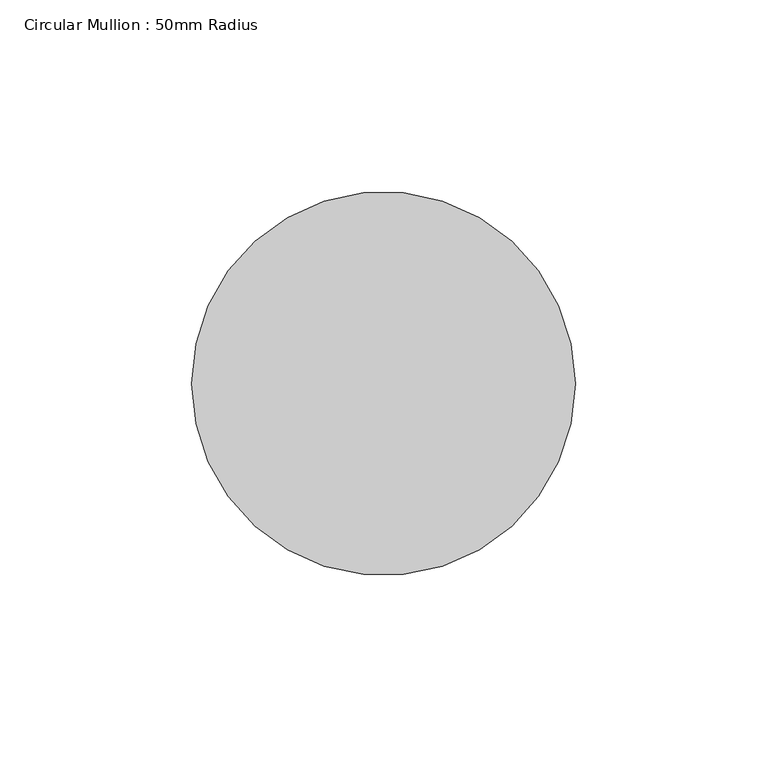
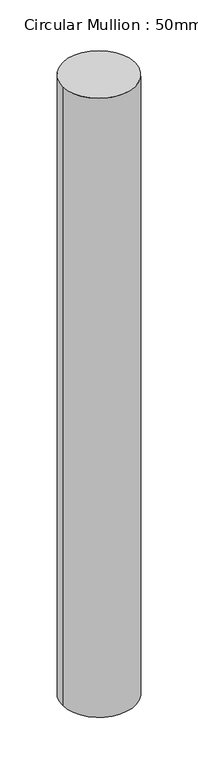
"""IFC4 building model written with IfcOpenShell, lengths in millimetres: member geometry, Circular Mullion : 50mm Radius."""

import ifcopenshell
import ifcopenshell.guid

model = None  # the IFC model being written
_history = None  # IfcOwnerHistory: only IFC2X3 demands one
_inside = {}  # id of a spatial element -> (the spatial element, [elements in it])
_under = {}  # id of a project, library or spatial element -> (it, [spatial elements below it])
_declared = {}  # id of a project -> (the project, [libraries it declares])
_typed = {}  # id of a type object -> (the type object, [elements of that type])
_made_of = {}  # id of a material, layer set ... -> (it, [elements and type objects made of it])


def new_model(schema):
    """Start an empty IFC model of exactly this schema.

    Asked for "IFC4X3", IfcOpenShell would pick the latest addendum, in which some entities
    have other attributes; the version numbers below select the first issue.
    IFC2X3 requires an IfcOwnerHistory on every rooted entity: one is made here for all.
    """
    global model, _history
    if schema == "IFC4X3":
        model = ifcopenshell.file(schema_version=(4, 3, 0, 0))
    else:
        model = ifcopenshell.file(schema=schema)
    _inside.clear()
    _under.clear()
    _declared.clear()
    _typed.clear()
    _made_of.clear()
    _history = None
    if model.schema == "IFC2X3":
        org = make("IfcOrganization", Name="unknown")
        user = make(
            "IfcPersonAndOrganization",
            ThePerson=make("IfcPerson", FamilyName="unknown"),
            TheOrganization=org,
        )
        app = make(
            "IfcApplication",
            ApplicationDeveloper=org,
            Version="unknown",
            ApplicationFullName="unknown",
            ApplicationIdentifier="unknown",
        )
        _history = make(
            "IfcOwnerHistory",
            OwningUser=user,
            OwningApplication=app,
            ChangeAction="ADDED",
            CreationDate=0,
        )
    return model


def make(cls, **values):
    """One entity of the class cls with the attributes given. An attribute that is None is left unset."""
    return model.create_entity(
        cls, **{name: value for name, value in values.items() if value is not None}
    )


def rooted(cls, **values):
    """An entity with a GlobalId (a new one), such as an element, a storey or a relation."""
    return make(cls, GlobalId=ifcopenshell.guid.new(), OwnerHistory=_history, **values)


def si_unit(unit_type, name, prefix=None):
    """IfcSIUnit, for example si_unit("LENGTHUNIT", "METRE", prefix="MILLI")."""
    return make("IfcSIUnit", UnitType=unit_type, Prefix=prefix, Name=name)


def assignment(units):
    """IfcUnitAssignment: the units of a project."""
    return None if units is None else make("IfcUnitAssignment", Units=units)


def point(xyz):
    """IfcCartesianPoint."""
    return None if xyz is None else make("IfcCartesianPoint", Coordinates=xyz)


def direction(xyz):
    """IfcDirection."""
    return None if xyz is None else make("IfcDirection", DirectionRatios=xyz)


def frame(location, z_axis=None, x_axis=None):
    """IfcAxis2Placement3D, a coordinate frame: its origin and axes. An axis left out is left unset."""
    return make(
        "IfcAxis2Placement3D",
        Location=point(location),
        Axis=direction(z_axis),
        RefDirection=direction(x_axis),
    )


def frame_2d(location, x_axis=None):
    """IfcAxis2Placement2D, a coordinate frame in the plane: its origin and x axis."""
    return make(
        "IfcAxis2Placement2D", Location=point(location), RefDirection=direction(x_axis)
    )


def origin():
    """The frame at (0, 0, 0) with its axes left unset."""
    return frame((0.0, 0.0, 0.0))


def origin_2d():
    """The frame at (0, 0) in the plane with its x axis left unset."""
    return frame_2d((0.0, 0.0))


def place(relative_to, where):
    """IfcLocalPlacement: puts the frame where relative to a parent placement (None: the world)."""
    return make(
        "IfcLocalPlacement", PlacementRelTo=relative_to, RelativePlacement=where
    )


def context(
    kind, dimensions, precision=None, world=None, true_north=None, identifier=None
):
    """IfcGeometricRepresentationContext, for example the 3D "Model" context."""
    return make(
        "IfcGeometricRepresentationContext",
        ContextIdentifier=identifier,
        ContextType=kind,
        CoordinateSpaceDimension=dimensions,
        Precision=precision,
        WorldCoordinateSystem=world,
        TrueNorth=true_north,
    )


def project(units=None, contexts=None):
    """IfcProject with its units and contexts."""
    return rooted(
        "IfcProject",
        Name="project",
        RepresentationContexts=contexts,
        UnitsInContext=assignment(units),
    )


def spatial(cls, under=None, at=None, **own):
    """A site, building, storey or space (cls), placed at a placement, below another one or the project."""
    s = rooted(cls, ObjectPlacement=at, **own)
    if under is not None:
        _under.setdefault(under.id(), (under, []))[1].append(s)
    return s


def circle_curve(where, radius):
    """IfcCircle in the frame where."""
    return make("IfcCircle", Position=where, Radius=radius)


def trimmed(basis, trim1, trim2, sense, master):
    """IfcTrimmedCurve: the piece of a basis curve between two trims."""
    return make(
        "IfcTrimmedCurve",
        BasisCurve=basis,
        Trim1=trim1,
        Trim2=trim2,
        SenseAgreement=sense,
        MasterRepresentation=master,
    )


def segment(curve, same_sense, transition):
    """IfcCompositeCurveSegment."""
    return make(
        "IfcCompositeCurveSegment",
        Transition=transition,
        SameSense=same_sense,
        ParentCurve=curve,
    )


def composite_curve(segments, self_intersect=None):
    """IfcCompositeCurve: segments joined end to end."""
    return make("IfcCompositeCurve", Segments=segments, SelfIntersect=self_intersect)


def outline(outer, holes=None, kind="AREA"):
    """IfcArbitraryClosedProfileDef: a profile drawn as a closed curve; with holes, ...WithVoids."""
    if holes is None:
        return make("IfcArbitraryClosedProfileDef", ProfileType=kind, OuterCurve=outer)
    return make(
        "IfcArbitraryProfileDefWithVoids",
        ProfileType=kind,
        OuterCurve=outer,
        InnerCurves=holes,
    )


def extrude(swept, where, along, depth):
    """IfcExtrudedAreaSolid: the profile swept, set in the frame where, extruded along a direction by depth."""
    return make(
        "IfcExtrudedAreaSolid",
        SweptArea=swept,
        Position=where,
        ExtrudedDirection=direction(along),
        Depth=depth,
    )


def shape(context_of_items, identifier, shape_type, items):
    """IfcShapeRepresentation: the items that make up one representation, for example the "Body"."""
    return make(
        "IfcShapeRepresentation",
        ContextOfItems=context_of_items,
        RepresentationIdentifier=identifier,
        RepresentationType=shape_type,
        Items=items,
    )


def source(mapping_origin, context_of_items, identifier, shape_type, items):
    """IfcRepresentationMap: a shape defined once, which mapped items show again and again."""
    return make(
        "IfcRepresentationMap",
        MappingOrigin=mapping_origin,
        MappedRepresentation=shape(context_of_items, identifier, shape_type, items),
    )


def transform(
    local_origin,
    x_axis=None,
    y_axis=None,
    z_axis=None,
    scale=None,
    scale2=None,
    scale3=None,
    uniform=True,
):
    """IfcCartesianTransformationOperator3D, or its non-uniform kind. x_axis, y_axis, z_axis: its Axis1, 2, 3."""
    if uniform:
        return make(
            "IfcCartesianTransformationOperator3D",
            Axis1=direction(x_axis),
            Axis2=direction(y_axis),
            LocalOrigin=point(local_origin),
            Scale=scale,
            Axis3=direction(z_axis),
        )
    return make(
        "IfcCartesianTransformationOperator3DnonUniform",
        Axis1=direction(x_axis),
        Axis2=direction(y_axis),
        LocalOrigin=point(local_origin),
        Scale=scale,
        Axis3=direction(z_axis),
        Scale2=scale2,
        Scale3=scale3,
    )


def mapped(mapping_source, mapping_target):
    """IfcMappedItem: shows the shape of a source again, moved by a transform."""
    return make(
        "IfcMappedItem", MappingSource=mapping_source, MappingTarget=mapping_target
    )


def made_of(thing, what):
    """Note that an element or type object is made of a material, layer set ...; save() writes the relation."""
    if what is not None:
        _made_of.setdefault(what.id(), (what, []))[1].append(thing)
    return thing


def element(
    cls,
    number,
    at=None,
    inside=None,
    cuts=None,
    type_object=None,
    material=None,
    context=None,
    identifier="Body",
    shape_type=None,
    held_by="IfcProductDefinitionShape",
    body=None,
    shapes=None,
    **own,
):
    """One element of the class cls, such as IfcWall. Its Tag is "e" and its number.

    at: its placement. inside: the storey or other place that contains it. cuts: it is an
    opening in that element (IfcRelVoidsElement). A single representation is given by context,
    identifier, shape_type and body (its items); several are given by shapes. held_by: the class
    of the entity that holds the representations. save() writes the other relations.
    """
    e = rooted(cls, Tag="e%d" % number, ObjectPlacement=at, **own)
    if body is not None:
        shapes = [shape(context, identifier, shape_type, body)]
    if shapes is not None:
        e.Representation = make(held_by, Representations=shapes)
    if inside is not None:
        _inside.setdefault(inside.id(), (inside, []))[1].append(e)
    if cuts is not None:
        rooted(
            "IfcRelVoidsElement", RelatingBuildingElement=cuts, RelatedOpeningElement=e
        )
    if type_object is not None:
        _typed.setdefault(type_object.id(), (type_object, []))[1].append(e)
    return made_of(e, material)


def aggregate(whole, parts):
    """IfcRelAggregates: a whole, such as a stair, and the parts it consists of."""
    return rooted("IfcRelAggregates", RelatingObject=whole, RelatedObjects=parts)


def save(model, path):
    """Write the relations noted so far, then the file.

    IfcRelAggregates (storeys below a building ...), IfcRelContainedInSpatialStructure (elements
    in a storey), IfcRelDefinesByType, IfcRelAssociatesMaterial and IfcRelDeclares: one each for
    every whole, place, type object, material and project.
    """
    for whole, parts in _under.values():
        aggregate(whole, parts)
    for where, things in _inside.values():
        rooted(
            "IfcRelContainedInSpatialStructure",
            RelatedElements=things,
            RelatingStructure=where,
        )
    for kind, things in _typed.values():
        rooted("IfcRelDefinesByType", RelatedObjects=things, RelatingType=kind)
    for what, things in _made_of.values():
        rooted("IfcRelAssociatesMaterial", RelatedObjects=things, RelatingMaterial=what)
    for by, libraries in _declared.values():
        rooted("IfcRelDeclares", RelatingContext=by, RelatedDefinitions=libraries)
    model.write(path)


def circular_mullion_50mm_radius_02db4220(model_context):
    return source(origin(), model_context, "Body", "SweptSolid", [
        extrude(outline(composite_curve([segment(trimmed(circle_curve(origin_2d(), 50.0), [point((50.0, 0.0))], [point((-50.0, 0.0))], False, "CARTESIAN"), True, "CONTINUOUS"), segment(trimmed(circle_curve(origin_2d(), 50.0), [point((-50.0, 0.0))], [point((50.0, 0.0))], False, "CARTESIAN"), True, "CONTINUOUS")], self_intersect=False)), frame((0.0, 0.0, -904.1337855), z_axis=(0.0, 0.0, 1.0), x_axis=(1.0, 0.0, 0.0)), (0.0, 0.0, 1.0), 904.1337855),
    ])


if __name__ == "__main__":
    model = new_model("IFC4")
    model_context = context("Model", 3, world=origin())
    ifc_project = project(units=[si_unit("LENGTHUNIT", "METRE", prefix="MILLI")], contexts=[model_context])
    site = spatial("IfcSite", under=ifc_project)
    building = spatial("IfcBuilding", under=site)
    placement = place(None, origin())
    circular_mullion_50mm_radius_shape = circular_mullion_50mm_radius_02db4220(model_context)
    element("IfcMember", 1, ObjectType="Circular Mullion : 50mm Radius", at=placement, inside=building, context=model_context, shape_type="MappedRepresentation", body=[
        mapped(circular_mullion_50mm_radius_shape, transform((0.0, 0.0, 0.0), x_axis=(1.0, 0.0, 0.0), y_axis=(0.0, 1.0, 0.0), z_axis=(0.0, 0.0, 1.0))),
    ])
    save(model, "model.ifc")

# Revit data of these elements
# Type "Circular Mullion : 50mm Radius"
#   built-in parameter 1007350 = 0.164042 (stored number, unit not read)
# Element 1 (IfcMember, "Circular Mullion : 50mm Radius")
#   Materials on its faces: "Aluminium"
# Materials
#   "Aluminium": class "Metal", colour RGB 247 247 247, transparency 0, Description = "Aluminium 6061", Cost = 0
